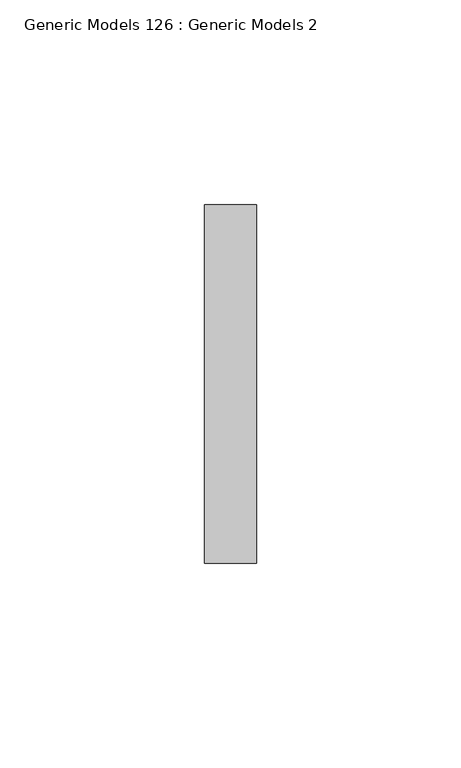
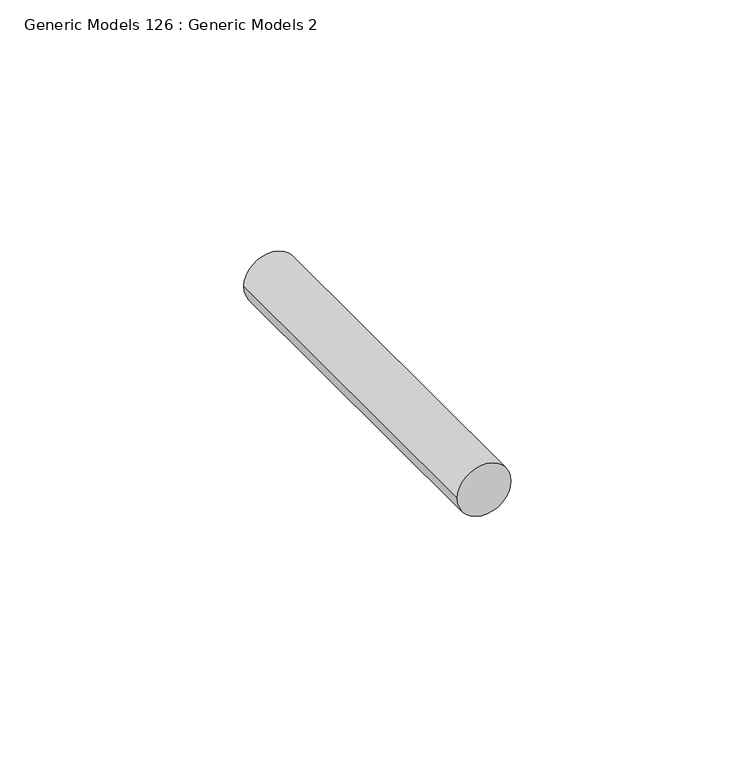
"""IFC4 building model written with IfcOpenShell, lengths in millimetres: proxy geometry, Generic Models 126 : Generic Models 2."""

from ifc_helpers import new_model, si_unit, point, frame, frame_2d, origin, place, context, project, spatial, circle_curve, trimmed, segment, composite_curve, outline, extrude, source, transform, mapped, element, save


def generic_models_126_generic_models_2_72507400(model_context):
    return source(origin(), model_context, "Body", "SweptSolid", [
        extrude(outline(composite_curve([segment(trimmed(circle_curve(frame_2d((38374.9548538, 7686.9828124)), 6.35), [point((38374.9548538, 7680.6328124))], [point((38374.9548538, 7693.3328124))], False, "CARTESIAN"), True, "CONTINUOUS"), segment(trimmed(circle_curve(frame_2d((38374.9548538, 7686.9828124)), 6.35), [point((38374.9548538, 7693.3328124))], [point((38374.9548538, 7680.6328124))], False, "CARTESIAN"), True, "CONTINUOUS")], self_intersect=False)), frame((0.0, 1848.3666731, 0.0), z_axis=(0.0, 1.0, 0.0), x_axis=(0.0, 0.0, 1.0)), (0.0, 0.0, 1.0), 87.551022),
    ])


if __name__ == "__main__":
    model = new_model("IFC4")
    model_context = context("Model", 3, world=origin())
    ifc_project = project(units=[si_unit("LENGTHUNIT", "METRE", prefix="MILLI")], contexts=[model_context])
    site = spatial("IfcSite", under=ifc_project)
    building = spatial("IfcBuilding", under=site)
    placement = place(None, origin())
    generic_models_126_generic_models_2_shape = generic_models_126_generic_models_2_72507400(model_context)
    element("IfcBuildingElementProxy", 1, Name="Generic Models 126 : Generic Models 2", ObjectType="Generic Models 126 : Generic Models 2", at=placement, inside=building, context=model_context, shape_type="MappedRepresentation", body=[
        mapped(generic_models_126_generic_models_2_shape, transform((0.0, 0.0, 0.0), x_axis=(1.0, 0.0, 0.0), y_axis=(0.0, 1.0, 0.0), z_axis=(0.0, 0.0, 1.0))),
    ])
    save(model, "model.ifc")

# Revit data of these elements
# Element 1 (IfcBuildingElementProxy, "Generic Models 126 : Generic Models 2")
#   Materials on its faces: "S.S. LAG BOLT - SEE STRUCT. DWGS"
# Materials
#   "S.S. LAG BOLT - SEE STRUCT. DWGS": class "Generic", colour RGB 120 120 120, transparency 0, Cost = 0
